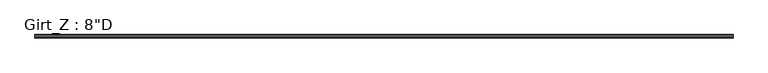
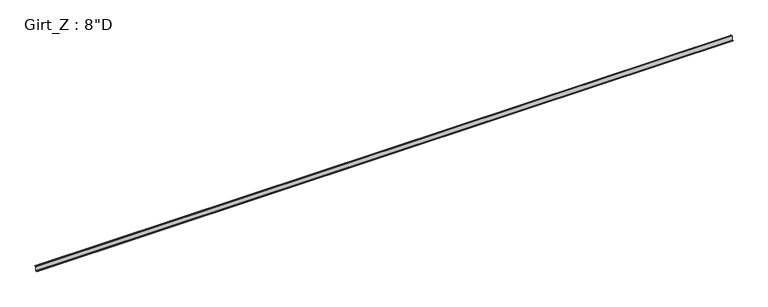
"""IFC4 building model written with IfcOpenShell, lengths in millimetres: beam geometry."""

from ifc_helpers import new_model, si_unit, point, frame, frame_2d, origin, place, context, project, spatial, polyline, circle_curve, trimmed, segment, composite_curve, outline, extrude, source, transform, mapped, element, save


def beam_221b0eb9(model_context):
    return source(origin(), model_context, "Body", "SweptSolid", [
        extrude(outline(composite_curve([segment(polyline([(63.5, 101.6), (75.745104, 87.0068534), (73.6169367, 85.221109), (62.204539, 98.821875), (3.3005807, 98.821875)]), True, "CONTINUOUS"), segment(trimmed(circle_curve(frame_2d((3.3741066, 96.8381931)), 1.9850441), [point((3.3005807, 98.821875))], [point((1.3890625, 96.8381931))], True, "CARTESIAN"), True, "CONTINUOUS"), segment(polyline([(1.3890625, 96.8381931), (1.3890625, -96.8375)]), True, "CONTINUOUS"), segment(trimmed(circle_curve(frame_2d((-3.3734375, -96.8375)), 4.7625), [point((1.3890625, -96.8375))], [point((-3.3734375, -101.6))], False, "CARTESIAN"), True, "CONTINUOUS"), segment(polyline([(-3.3734375, -101.6), (-63.5, -101.6), (-75.745104, -87.0068534), (-73.6169367, -85.221109), (-62.204539, -98.821875), (-3.2694106, -98.821875)]), True, "CONTINUOUS"), segment(trimmed(circle_curve(frame_2d((-3.3748024, -96.8389339)), 1.9857399), [point((-3.2694106, -98.821875))], [point((-1.3890625, -96.8389339))], True, "CARTESIAN"), True, "CONTINUOUS"), segment(polyline([(-1.3890625, -96.8389339), (-1.3890625, 96.8375)]), True, "CONTINUOUS"), segment(trimmed(circle_curve(frame_2d((3.3734375, 96.8375)), 4.7625), [point((-1.3890625, 96.8375))], [point((3.3734375, 101.6))], False, "CARTESIAN"), True, "CONTINUOUS"), segment(polyline([(3.3734375, 101.6), (63.5, 101.6)]), True, "CONTINUOUS")], self_intersect=False)), frame((-15623.38125, 0.0, 0.0), z_axis=(1.0, 0.0, 0.0), x_axis=(0.0, 1.0, 0.0)), (0.0, 0.0, 1.0), 31246.7625),
    ])


if __name__ == "__main__":
    model = new_model("IFC4")
    model_context = context("Model", 3, world=origin())
    ifc_project = project(units=[si_unit("LENGTHUNIT", "METRE", prefix="MILLI")], contexts=[model_context])
    site = spatial("IfcSite", under=ifc_project)
    building = spatial("IfcBuilding", under=site)
    placement = place(None, origin())
    beam_shape = beam_221b0eb9(model_context)
    element("IfcBeam", 1, ObjectType="Girt_Z : 8\"D", at=placement, inside=building, context=model_context, shape_type="MappedRepresentation", body=[
        mapped(beam_shape, transform((0.0, 0.0, 0.0), x_axis=(1.0, 0.0, 0.0), y_axis=(0.0, 1.0, 0.0), z_axis=(0.0, 0.0, 1.0))),
    ])
    save(model, "model.ifc")

# Revit data of these elements
# Type "Girt_Z : 8\"D"
#   Web_Thickness = 0' - 0 7/64"
#   Length [instance default] = 10' - 0"
#   Leg_1 = 0' - 2 1/2"
#   Height = 0' - 8"
#   Structural Material [instance default] = none
# Element 1 (IfcBeam, "Girt_Z : 8\"D")
#   Structural Material = Steel
#   Materials on its faces: "Steel"
# Materials
#   "Steel": class "Metal", colour RGB 118 118 114, transparency 0, Description = "Steel, mill finish", Cost = 0
